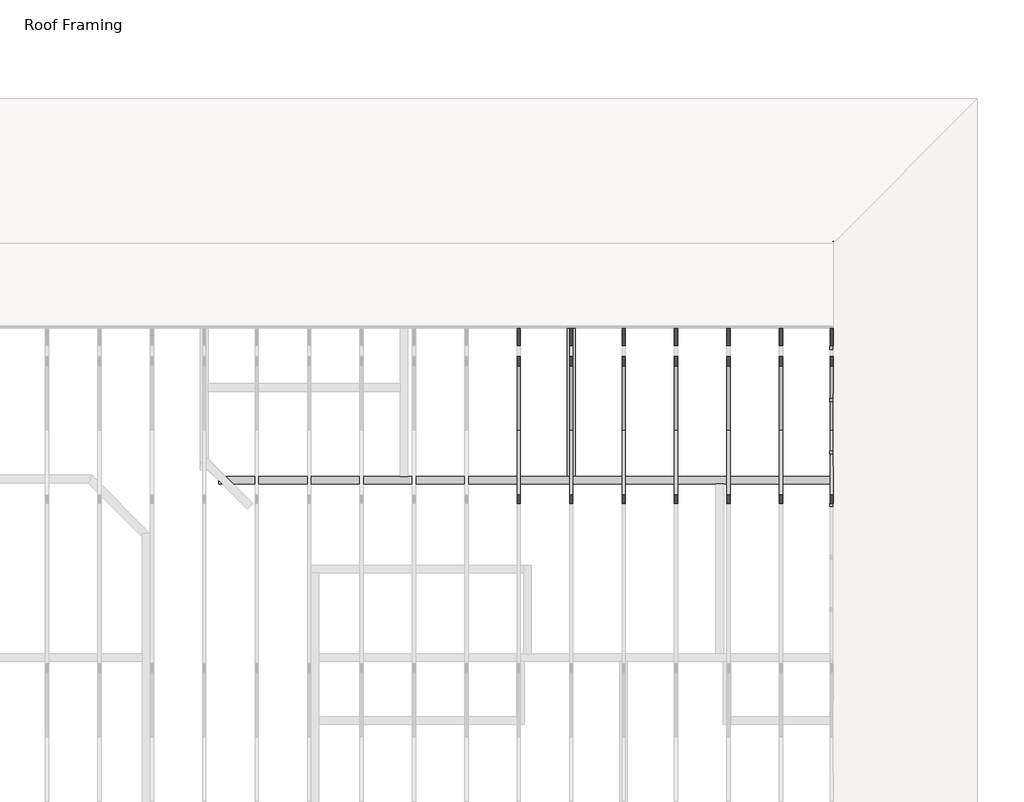
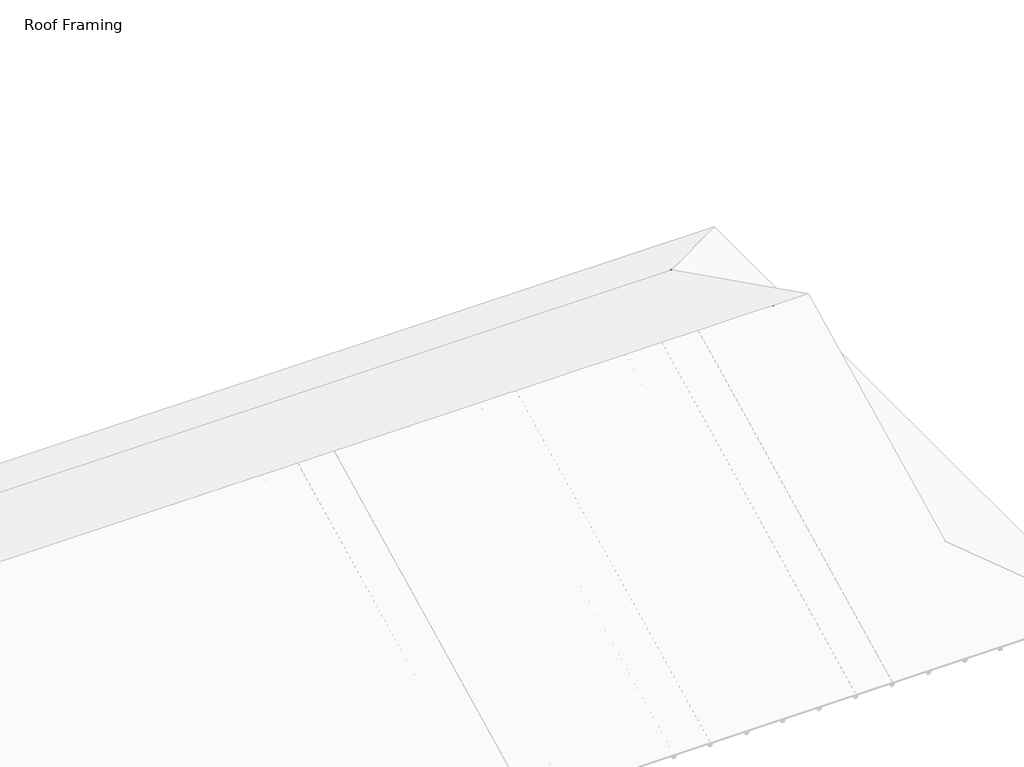
# One storey, part 7 of 7: 46 beams, 14 members.
"""IFC4 building model written with IfcOpenShell, lengths in millimetres."""

import ifcopenshell
import ifcopenshell.guid

model = None  # the IFC model being written
_history = None  # IfcOwnerHistory: only IFC2X3 demands one
_inside = {}  # id of a spatial element -> (the spatial element, [elements in it])
_under = {}  # id of a project, library or spatial element -> (it, [spatial elements below it])
_declared = {}  # id of a project -> (the project, [libraries it declares])
_typed = {}  # id of a type object -> (the type object, [elements of that type])
_made_of = {}  # id of a material, layer set ... -> (it, [elements and type objects made of it])


def new_model(schema):
    """Start an empty IFC model of exactly this schema.

    Asked for "IFC4X3", IfcOpenShell would pick the latest addendum, in which some entities
    have other attributes; the version numbers below select the first issue.
    IFC2X3 requires an IfcOwnerHistory on every rooted entity: one is made here for all.
    """
    global model, _history
    if schema == "IFC4X3":
        model = ifcopenshell.file(schema_version=(4, 3, 0, 0))
    else:
        model = ifcopenshell.file(schema=schema)
    _inside.clear()
    _under.clear()
    _declared.clear()
    _typed.clear()
    _made_of.clear()
    _history = None
    if model.schema == "IFC2X3":
        org = make("IfcOrganization", Name="unknown")
        user = make(
            "IfcPersonAndOrganization",
            ThePerson=make("IfcPerson", FamilyName="unknown"),
            TheOrganization=org,
        )
        app = make(
            "IfcApplication",
            ApplicationDeveloper=org,
            Version="unknown",
            ApplicationFullName="unknown",
            ApplicationIdentifier="unknown",
        )
        _history = make(
            "IfcOwnerHistory",
            OwningUser=user,
            OwningApplication=app,
            ChangeAction="ADDED",
            CreationDate=0,
        )
    return model


def make(cls, **values):
    """One entity of the class cls with the attributes given. An attribute that is None is left unset."""
    return model.create_entity(
        cls, **{name: value for name, value in values.items() if value is not None}
    )


def rooted(cls, **values):
    """An entity with a GlobalId (a new one), such as an element, a storey or a relation."""
    return make(cls, GlobalId=ifcopenshell.guid.new(), OwnerHistory=_history, **values)


def si_unit(unit_type, name, prefix=None):
    """IfcSIUnit, for example si_unit("LENGTHUNIT", "METRE", prefix="MILLI")."""
    return make("IfcSIUnit", UnitType=unit_type, Prefix=prefix, Name=name)


def assignment(units):
    """IfcUnitAssignment: the units of a project."""
    return None if units is None else make("IfcUnitAssignment", Units=units)


def point(xyz):
    """IfcCartesianPoint."""
    return None if xyz is None else make("IfcCartesianPoint", Coordinates=xyz)


def direction(xyz):
    """IfcDirection."""
    return None if xyz is None else make("IfcDirection", DirectionRatios=xyz)


def frame(location, z_axis=None, x_axis=None):
    """IfcAxis2Placement3D, a coordinate frame: its origin and axes. An axis left out is left unset."""
    return make(
        "IfcAxis2Placement3D",
        Location=point(location),
        Axis=direction(z_axis),
        RefDirection=direction(x_axis),
    )


def origin():
    """The frame at (0, 0, 0) with its axes left unset."""
    return frame((0.0, 0.0, 0.0))


def place(relative_to, where):
    """IfcLocalPlacement: puts the frame where relative to a parent placement (None: the world)."""
    return make(
        "IfcLocalPlacement", PlacementRelTo=relative_to, RelativePlacement=where
    )


def context(
    kind, dimensions, precision=None, world=None, true_north=None, identifier=None
):
    """IfcGeometricRepresentationContext, for example the 3D "Model" context."""
    return make(
        "IfcGeometricRepresentationContext",
        ContextIdentifier=identifier,
        ContextType=kind,
        CoordinateSpaceDimension=dimensions,
        Precision=precision,
        WorldCoordinateSystem=world,
        TrueNorth=true_north,
    )


def project(units=None, contexts=None):
    """IfcProject with its units and contexts."""
    return rooted(
        "IfcProject",
        Name="project",
        RepresentationContexts=contexts,
        UnitsInContext=assignment(units),
    )


def spatial(cls, under=None, at=None, **own):
    """A site, building, storey or space (cls), placed at a placement, below another one or the project."""
    s = rooted(cls, ObjectPlacement=at, **own)
    if under is not None:
        _under.setdefault(under.id(), (under, []))[1].append(s)
    return s


def polyline(points):
    """IfcPolyline through the points."""
    return make("IfcPolyline", Points=[point(p) for p in points])


def outline(outer, holes=None, kind="AREA"):
    """IfcArbitraryClosedProfileDef: a profile drawn as a closed curve; with holes, ...WithVoids."""
    if holes is None:
        return make("IfcArbitraryClosedProfileDef", ProfileType=kind, OuterCurve=outer)
    return make(
        "IfcArbitraryProfileDefWithVoids",
        ProfileType=kind,
        OuterCurve=outer,
        InnerCurves=holes,
    )


def extrude(swept, where, along, depth):
    """IfcExtrudedAreaSolid: the profile swept, set in the frame where, extruded along a direction by depth."""
    return make(
        "IfcExtrudedAreaSolid",
        SweptArea=swept,
        Position=where,
        ExtrudedDirection=direction(along),
        Depth=depth,
    )


def shape(context_of_items, identifier, shape_type, items):
    """IfcShapeRepresentation: the items that make up one representation, for example the "Body"."""
    return make(
        "IfcShapeRepresentation",
        ContextOfItems=context_of_items,
        RepresentationIdentifier=identifier,
        RepresentationType=shape_type,
        Items=items,
    )


def source(mapping_origin, context_of_items, identifier, shape_type, items):
    """IfcRepresentationMap: a shape defined once, which mapped items show again and again."""
    return make(
        "IfcRepresentationMap",
        MappingOrigin=mapping_origin,
        MappedRepresentation=shape(context_of_items, identifier, shape_type, items),
    )


def transform(
    local_origin,
    x_axis=None,
    y_axis=None,
    z_axis=None,
    scale=None,
    scale2=None,
    scale3=None,
    uniform=True,
):
    """IfcCartesianTransformationOperator3D, or its non-uniform kind. x_axis, y_axis, z_axis: its Axis1, 2, 3."""
    if uniform:
        return make(
            "IfcCartesianTransformationOperator3D",
            Axis1=direction(x_axis),
            Axis2=direction(y_axis),
            LocalOrigin=point(local_origin),
            Scale=scale,
            Axis3=direction(z_axis),
        )
    return make(
        "IfcCartesianTransformationOperator3DnonUniform",
        Axis1=direction(x_axis),
        Axis2=direction(y_axis),
        LocalOrigin=point(local_origin),
        Scale=scale,
        Axis3=direction(z_axis),
        Scale2=scale2,
        Scale3=scale3,
    )


def mapped(mapping_source, mapping_target):
    """IfcMappedItem: shows the shape of a source again, moved by a transform."""
    return make(
        "IfcMappedItem", MappingSource=mapping_source, MappingTarget=mapping_target
    )


def made_of(thing, what):
    """Note that an element or type object is made of a material, layer set ...; save() writes the relation."""
    if what is not None:
        _made_of.setdefault(what.id(), (what, []))[1].append(thing)
    return thing


def element(
    cls,
    number,
    at=None,
    inside=None,
    cuts=None,
    type_object=None,
    material=None,
    context=None,
    identifier="Body",
    shape_type=None,
    held_by="IfcProductDefinitionShape",
    body=None,
    shapes=None,
    **own,
):
    """One element of the class cls, such as IfcWall. Its Tag is "e" and its number.

    at: its placement. inside: the storey or other place that contains it. cuts: it is an
    opening in that element (IfcRelVoidsElement). A single representation is given by context,
    identifier, shape_type and body (its items); several are given by shapes. held_by: the class
    of the entity that holds the representations. save() writes the other relations.
    """
    e = rooted(cls, Tag="e%d" % number, ObjectPlacement=at, **own)
    if body is not None:
        shapes = [shape(context, identifier, shape_type, body)]
    if shapes is not None:
        e.Representation = make(held_by, Representations=shapes)
    if inside is not None:
        _inside.setdefault(inside.id(), (inside, []))[1].append(e)
    if cuts is not None:
        rooted(
            "IfcRelVoidsElement", RelatingBuildingElement=cuts, RelatedOpeningElement=e
        )
    if type_object is not None:
        _typed.setdefault(type_object.id(), (type_object, []))[1].append(e)
    return made_of(e, material)


def aggregate(whole, parts):
    """IfcRelAggregates: a whole, such as a stair, and the parts it consists of."""
    return rooted("IfcRelAggregates", RelatingObject=whole, RelatedObjects=parts)


def save(model, path):
    """Write the relations noted so far, then the file.

    IfcRelAggregates (storeys below a building ...), IfcRelContainedInSpatialStructure (elements
    in a storey), IfcRelDefinesByType, IfcRelAssociatesMaterial and IfcRelDeclares: one each for
    every whole, place, type object, material and project.
    """
    for whole, parts in _under.values():
        aggregate(whole, parts)
    for where, things in _inside.values():
        rooted(
            "IfcRelContainedInSpatialStructure",
            RelatedElements=things,
            RelatingStructure=where,
        )
    for kind, things in _typed.values():
        rooted("IfcRelDefinesByType", RelatedObjects=things, RelatingType=kind)
    for what, things in _made_of.values():
        rooted("IfcRelAssociatesMaterial", RelatedObjects=things, RelatingMaterial=what)
    for by, libraries in _declared.values():
        rooted("IfcRelDeclares", RelatingContext=by, RelatedDefinitions=libraries)
    model.write(path)


def dimension_lumber_72c26da1(model_context):
    return source(origin(), model_context, "Body", "SweptSolid", [
        extrude(outline(polyline([(927.1, 44.45), (927.1, -44.45), (-971.55, -44.45), (-971.55, 44.45), (927.1, 44.45)])), frame((0.0, 0.0, -19.05), z_axis=(0.0, 0.0, 1.0), x_axis=(1.0, 0.0, 0.0)), (0.0, 0.0, 1.0), 38.1),
    ])


def dimension_lumber_1b552245(model_context):
    return source(origin(), model_context, "Body", "SweptSolid", [
        extrude(outline(polyline([(1918.49375, 44.45), (1918.49375, -44.45), (-1918.49375, -44.45), (-1918.49375, 44.45), (1918.49375, 44.45)])), frame((0.0, 0.0, -19.05), z_axis=(0.0, 0.0, 1.0), x_axis=(1.0, 0.0, 0.0)), (0.0, 0.0, 1.0), 38.1),
    ])


def dimension_lumber_5c8890d8(model_context):
    return source(origin(), model_context, "Body", "SweptSolid", [
        extrude(outline(polyline([(330.0062925, 44.45), (330.0062925, -44.45), (-285.5562925, -44.45), (-285.5562925, 44.45), (330.0062925, 44.45)])), frame((0.0, 0.0, -19.05), z_axis=(0.0, 0.0, 1.0), x_axis=(1.0, 0.0, 0.0)), (0.0, 0.0, 1.0), 38.1),
    ])


def dimension_lumber_f00769ea(model_context):
    return source(origin(), model_context, "Body", "SweptSolid", [
        extrude(outline(polyline([(927.1, 44.45), (927.1, -44.45), (-1016.0, -44.45), (-1016.0, 44.45), (927.1, 44.45)])), frame((0.0, 0.0, -19.05), z_axis=(0.0, 0.0, 1.0), x_axis=(1.0, 0.0, 0.0)), (0.0, 0.0, 1.0), 38.1),
    ])


def dimension_lumber_39962a34(model_context):
    return source(origin(), model_context, "Body", "SweptSolid", [
        extrude(outline(polyline([(1941.5125, 44.45), (1941.5125, -44.45), (-1895.475, -44.45), (-1895.475, 44.45), (1941.5125, 44.45)])), frame((0.0, 0.0, -19.05), z_axis=(0.0, 0.0, 1.0), x_axis=(1.0, 0.0, 0.0)), (0.0, 0.0, 1.0), 38.1),
    ])


def dimension_lumber_4fd1e5d7(model_context):
    return source(origin(), model_context, "Body", "SweptSolid", [
        extrude(outline(polyline([(285.5562925, 44.45), (285.5562925, -44.45), (-330.0062925, -44.45), (-330.0062925, 44.45), (285.5562925, 44.45)])), frame((0.0, 0.0, -19.05), z_axis=(0.0, 0.0, 1.0), x_axis=(1.0, 0.0, 0.0)), (0.0, 0.0, 1.0), 38.1),
    ])


model = new_model("IFC4")

# Units and contexts
model_context = context("Model", 3, world=origin())
ifc_project = project(units=[si_unit("LENGTHUNIT", "METRE", prefix="MILLI")], contexts=[model_context])

# Site, building, storey
site = spatial("IfcSite", under=ifc_project)
building = spatial("IfcBuilding", under=site)
storey = spatial("IfcBuildingStorey", under=building, Name="Roof Framing", Elevation=2768.6)

# Beams
placement = place(None, origin())
element("IfcBeam", 1, ObjectType="Dimension Lumber : Roof Lumbers", at=placement, inside=storey, context=model_context, shape_type="SweptSolid", body=[
    extrude(outline(polyline([(0.0, -38.1), (0.0, 0.0), (1874.2721787, 0.0), (1874.2721787, -38.1), (0.0, -38.1)])), frame((13672.6274862, 213.0959053, 2554.840297), z_axis=(0.44721359549993345, 0.0, 0.8944271909999282), x_axis=(-0.8944271909999282, 0.0, 0.44721359549993345)), (0.0, 0.0, 1.0), 88.9),
    extrude(outline(polyline([(2554.840297, 13672.6274862), (2558.1548743, 13674.2847749), (2653.4048743, 13674.2847749), (3472.5548743, 12035.9847749), (3393.040297, 11996.2274862), (2554.840297, 13672.6274862)])), frame((0.0, 213.0959053, 0.0), z_axis=(0.0, 1.0, 0.0), x_axis=(0.0, 0.0, 1.0)), (0.0, 0.0, 1.0), 38.1),
    extrude(outline(polyline([(2554.840297, 13672.6274862), (2558.1548743, 13674.2847749), (2653.4048743, 13674.2847749), (3472.5548743, 12035.9847749), (3373.1616527, 12035.9847749), (2554.840297, 13672.6274862)])), frame((0.0, 213.0959053, 0.0), z_axis=(0.0, 1.0, 0.0), x_axis=(0.0, 0.0, 1.0)), (0.0, 0.0, 1.0), 38.1),
])
element("IfcBeam", 2, ObjectType="Dimension Lumber : Roof Lumbers", at=placement, inside=storey, context=model_context, shape_type="SweptSolid", body=[
    extrude(outline(polyline([(0.0, -38.1), (0.0, 0.0), (1874.2721787, 0.0), (1874.2721787, -38.1), (0.0, -38.1)])), frame((13672.6274862, 822.6959053, 2554.840297), z_axis=(0.44721359549993367, 0.0, 0.8944271909999281), x_axis=(-0.8944271909999281, 0.0, 0.44721359549993367)), (0.0, 0.0, 1.0), 88.9),
    extrude(outline(polyline([(2554.840297, 13672.6274862), (2558.1548743, 13674.2847749), (2653.4048743, 13674.2847749), (3472.5548743, 12035.9847749), (3393.040297, 11996.2274862), (2554.840297, 13672.6274862)])), frame((0.0, 822.6959053, 0.0), z_axis=(0.0, 1.0, 0.0), x_axis=(0.0, 0.0, 1.0)), (0.0, 0.0, 1.0), 38.1),
    extrude(outline(polyline([(2554.840297, 13672.6274862), (2558.1548743, 13674.2847749), (2653.4048743, 13674.2847749), (3472.5548743, 12035.9847749), (3373.1616527, 12035.9847749), (2554.840297, 13672.6274862)])), frame((0.0, 822.6959053, 0.0), z_axis=(0.0, 1.0, 0.0), x_axis=(0.0, 0.0, 1.0)), (0.0, 0.0, 1.0), 38.1),
])
element("IfcBeam", 3, ObjectType="Dimension Lumber : Roof Lumbers", at=placement, inside=storey, context=model_context, shape_type="SweptSolid", body=[
    extrude(outline(polyline([(0.0, -38.1), (0.0, 0.0), (1874.2721787, 0.0), (1874.2721787, -38.1), (0.0, -38.1)])), frame((13672.6274862, 1432.2959053, 2554.840297), z_axis=(0.44721359549993367, 0.0, 0.8944271909999281), x_axis=(-0.8944271909999281, 0.0, 0.44721359549993367)), (0.0, 0.0, 1.0), 88.9),
    extrude(outline(polyline([(2554.840297, 13672.6274862), (2558.1548743, 13674.2847749), (2653.4048743, 13674.2847749), (3472.5548743, 12035.9847749), (3393.040297, 11996.2274862), (2554.840297, 13672.6274862)])), frame((0.0, 1432.2959053, 0.0), z_axis=(0.0, 1.0, 0.0), x_axis=(0.0, 0.0, 1.0)), (0.0, 0.0, 1.0), 38.1),
    extrude(outline(polyline([(2554.840297, 13672.6274862), (2558.1548743, 13674.2847749), (2653.4048743, 13674.2847749), (3472.5548743, 12035.9847749), (3373.1616527, 12035.9847749), (2554.840297, 13672.6274862)])), frame((0.0, 1432.2959053, 0.0), z_axis=(0.0, 1.0, 0.0), x_axis=(0.0, 0.0, 1.0)), (0.0, 0.0, 1.0), 38.1),
])
element("IfcBeam", 4, ObjectType="Dimension Lumber : Roof Lumbers", at=placement, inside=storey, context=model_context, shape_type="SweptSolid", body=[
    extrude(outline(polyline([(0.0, -38.1), (0.0, 0.0), (1874.2721787, 0.0), (1874.2721787, -38.1), (0.0, -38.1)])), frame((13672.6274862, 2041.8959053, 2554.840297), z_axis=(0.44721359549993345, 0.0, 0.8944271909999282), x_axis=(-0.8944271909999282, 0.0, 0.44721359549993345)), (0.0, 0.0, 1.0), 88.9),
    extrude(outline(polyline([(2554.840297, 13672.6274862), (2558.1548743, 13674.2847749), (2653.4048743, 13674.2847749), (3472.5548743, 12035.9847749), (3393.040297, 11996.2274862), (2554.840297, 13672.6274862)])), frame((0.0, 2041.8959053, 0.0), z_axis=(0.0, 1.0, 0.0), x_axis=(0.0, 0.0, 1.0)), (0.0, 0.0, 1.0), 38.1),
    extrude(outline(polyline([(2554.840297, 13672.6274862), (2558.1548743, 13674.2847749), (2653.4048743, 13674.2847749), (3472.5548743, 12035.9847749), (3373.1616527, 12035.9847749), (2554.840297, 13672.6274862)])), frame((0.0, 2041.8959053, 0.0), z_axis=(0.0, 1.0, 0.0), x_axis=(0.0, 0.0, 1.0)), (0.0, 0.0, 1.0), 38.1),
])
element("IfcBeam", 5, ObjectType="Dimension Lumber : Roof Lumbers", at=placement, inside=storey, context=model_context, shape_type="SweptSolid", body=[
    extrude(outline(polyline([(0.0, -38.1), (0.0, 0.0), (1874.2721787, 0.0), (1874.2721787, -38.1), (0.0, -38.1)])), frame((13672.6274862, 2651.4959053, 2554.840297), z_axis=(0.44721359549993367, 0.0, 0.8944271909999281), x_axis=(-0.8944271909999281, 0.0, 0.44721359549993367)), (0.0, 0.0, 1.0), 88.9),
    extrude(outline(polyline([(2554.840297, 13672.6274862), (2558.1548743, 13674.2847749), (2653.4048743, 13674.2847749), (3472.5548743, 12035.9847749), (3393.040297, 11996.2274862), (2554.840297, 13672.6274862)])), frame((0.0, 2651.4959053, 0.0), z_axis=(0.0, 1.0, 0.0), x_axis=(0.0, 0.0, 1.0)), (0.0, 0.0, 1.0), 38.1),
    extrude(outline(polyline([(2554.840297, 13672.6274862), (2558.1548743, 13674.2847749), (2653.4048743, 13674.2847749), (3472.5548743, 12035.9847749), (3373.1616527, 12035.9847749), (2554.840297, 13672.6274862)])), frame((0.0, 2651.4959053, 0.0), z_axis=(0.0, 1.0, 0.0), x_axis=(0.0, 0.0, 1.0)), (0.0, 0.0, 1.0), 38.1),
])
element("IfcBeam", 6, ObjectType="Dimension Lumber : Roof Lumbers", at=placement, inside=storey, context=model_context, shape_type="SweptSolid", body=[
    extrude(outline(polyline([(0.0, -38.1), (0.0, 0.0), (1877.070187, 0.0), (1877.070187, -38.1), (0.0, -38.1)])), frame((13672.6274862, 3261.0959053, 2554.840297), z_axis=(0.44721359549993367, 0.0, 0.8944271909999281), x_axis=(-0.8944271909999281, 0.0, 0.44721359549993367)), (0.0, 0.0, 1.0), 88.9),
    extrude(outline(polyline([(2554.840297, 13672.6274862), (2558.1548743, 13674.2847749), (2653.4048743, 13674.2847749), (3473.8061816, 12033.4821602), (3394.2916044, 11993.7248716), (2554.840297, 13672.6274862)])), frame((0.0, 3261.0959053, 0.0), z_axis=(0.0, 1.0, 0.0), x_axis=(0.0, 0.0, 1.0)), (0.0, 0.0, 1.0), 38.1),
    extrude(outline(polyline([(2554.840297, 13672.6274862), (2558.1548743, 13674.2847749), (2653.4048743, 13674.2847749), (3472.5548743, 12035.9847749), (3373.1616527, 12035.9847749), (2554.840297, 13672.6274862)])), frame((0.0, 3261.0959053, 0.0), z_axis=(0.0, 1.0, 0.0), x_axis=(0.0, 0.0, 1.0)), (0.0, 0.0, 1.0), 38.1),
])
element("IfcBeam", 7, ObjectType="Dimension Lumber : Roof Lumbers", at=placement, inside=storey, context=model_context, shape_type="SweptSolid", body=[
    extrude(outline(polyline([(12035.9847749, 251.1959053), (13244.0722749, 251.1959053), (13244.0722749, 213.0959053), (12035.9847749, 213.0959053), (12035.9847749, 251.1959053)])), frame((0.0, 0.0, 2768.6), z_axis=(0.0, 0.0, 1.0), x_axis=(1.0, 0.0, 0.0)), (0.0, 0.0, 1.0), 88.9),
    extrude(outline(polyline([(2768.6, 12035.9847749), (2768.6, 13244.0722749), (2769.1179027, 13244.0722749), (2857.5, 13067.3080803), (2857.5, 12035.9847749), (2768.6, 12035.9847749)])), frame((0.0, 213.0959053, 0.0), z_axis=(0.0, 1.0, 0.0), x_axis=(0.0, 0.0, 1.0)), (0.0, 0.0, 1.0), 38.1),
])
element("IfcBeam", 8, ObjectType="Dimension Lumber : Roof Lumbers", at=placement, inside=storey, context=model_context, shape_type="SweptSolid", body=[
    extrude(outline(polyline([(12035.9847749, 860.7959053), (13244.0722749, 860.7959053), (13244.0722749, 822.6959053), (12035.9847749, 822.6959053), (12035.9847749, 860.7959053)])), frame((0.0, 0.0, 2768.6), z_axis=(0.0, 0.0, 1.0), x_axis=(1.0, 0.0, 0.0)), (0.0, 0.0, 1.0), 88.9),
    extrude(outline(polyline([(2768.6, 12035.9847749), (2768.6, 13244.0722749), (2769.1179027, 13244.0722749), (2857.5, 13067.3080803), (2857.5, 12035.9847749), (2768.6, 12035.9847749)])), frame((0.0, 822.6959053, 0.0), z_axis=(0.0, 1.0, 0.0), x_axis=(0.0, 0.0, 1.0)), (0.0, 0.0, 1.0), 38.1),
])
element("IfcBeam", 9, ObjectType="Dimension Lumber : Roof Lumbers", at=placement, inside=storey, context=model_context, shape_type="SweptSolid", body=[
    extrude(outline(polyline([(12035.9847749, 1470.3959053), (13244.0722749, 1470.3959053), (13244.0722749, 1432.2959053), (12035.9847749, 1432.2959053), (12035.9847749, 1470.3959053)])), frame((0.0, 0.0, 2768.6), z_axis=(0.0, 0.0, 1.0), x_axis=(1.0, 0.0, 0.0)), (0.0, 0.0, 1.0), 88.9),
    extrude(outline(polyline([(2768.6, 12035.9847749), (2768.6, 13244.0722749), (2769.1179027, 13244.0722749), (2857.5, 13067.3080803), (2857.5, 12035.9847749), (2768.6, 12035.9847749)])), frame((0.0, 1432.2959053, 0.0), z_axis=(0.0, 1.0, 0.0), x_axis=(0.0, 0.0, 1.0)), (0.0, 0.0, 1.0), 38.1),
])
element("IfcBeam", 10, ObjectType="Dimension Lumber : Roof Lumbers", at=placement, inside=storey, context=model_context, shape_type="SweptSolid", body=[
    extrude(outline(polyline([(12035.9847749, 2079.9959053), (13244.0722749, 2079.9959053), (13244.0722749, 2041.8959053), (12035.9847749, 2041.8959053), (12035.9847749, 2079.9959053)])), frame((0.0, 0.0, 2768.6), z_axis=(0.0, 0.0, 1.0), x_axis=(1.0, 0.0, 0.0)), (0.0, 0.0, 1.0), 88.9),
    extrude(outline(polyline([(2768.6, 12035.9847749), (2768.6, 13244.0722749), (2769.1179027, 13244.0722749), (2857.5, 13067.3080803), (2857.5, 12035.9847749), (2768.6, 12035.9847749)])), frame((0.0, 2041.8959053, 0.0), z_axis=(0.0, 1.0, 0.0), x_axis=(0.0, 0.0, 1.0)), (0.0, 0.0, 1.0), 38.1),
])
element("IfcBeam", 11, ObjectType="Dimension Lumber : Roof Lumbers", at=placement, inside=storey, context=model_context, shape_type="SweptSolid", body=[
    extrude(outline(polyline([(12035.9847749, 2689.5959053), (13244.0722749, 2689.5959053), (13244.0722749, 2651.4959053), (12035.9847749, 2651.4959053), (12035.9847749, 2689.5959053)])), frame((0.0, 0.0, 2768.6), z_axis=(0.0, 0.0, 1.0), x_axis=(1.0, 0.0, 0.0)), (0.0, 0.0, 1.0), 88.9),
    extrude(outline(polyline([(2768.6, 12035.9847749), (2768.6, 13244.0722749), (2769.1179027, 13244.0722749), (2857.5, 13067.3080803), (2857.5, 12035.9847749), (2768.6, 12035.9847749)])), frame((0.0, 2651.4959053, 0.0), z_axis=(0.0, 1.0, 0.0), x_axis=(0.0, 0.0, 1.0)), (0.0, 0.0, 1.0), 38.1),
])
element("IfcBeam", 12, ObjectType="Dimension Lumber : Roof Lumbers", at=placement, inside=storey, context=model_context, shape_type="SweptSolid", body=[
    extrude(outline(polyline([(12035.9847749, 3299.1959053), (13244.0722749, 3299.1959053), (13244.0722749, 3261.0959053), (12035.9847749, 3261.0959053), (12035.9847749, 3299.1959053)])), frame((0.0, 0.0, 2768.6), z_axis=(0.0, 0.0, 1.0), x_axis=(1.0, 0.0, 0.0)), (0.0, 0.0, 1.0), 88.9),
    extrude(outline(polyline([(2768.6, 12035.9847749), (2768.6, 13244.0722749), (2769.1179027, 13244.0722749), (2857.5, 13067.3080803), (2857.5, 12035.9847749), (2768.6, 12035.9847749)])), frame((0.0, 3261.0959053, 0.0), z_axis=(0.0, 1.0, 0.0), x_axis=(0.0, 0.0, 1.0)), (0.0, 0.0, 1.0), 38.1),
])
element("IfcBeam", 13, ObjectType="Dimension Lumber : Top Supporting Lumbers", at=placement, inside=storey, context=model_context, shape_type="SweptSolid", body=[
    extrude(outline(polyline([(13155.1722749, 562.3459053), (13155.1722749, 473.4459053), (4885.8847749, 473.4459053), (4885.8847749, 562.3459053), (13155.1722749, 562.3459053)])), frame((0.0, 0.0, 2692.4), z_axis=(0.0, 0.0, 1.0), x_axis=(1.0, 0.0, 0.0)), (0.0, 0.0, 1.0), 38.1),
    extrude(outline(polyline([(13155.1722749, 562.3459053), (13155.1722749, 473.4459053), (4930.3347749, 473.4459053), (4967.1583606, 562.3459053), (13155.1722749, 562.3459053)])), frame((0.0, 0.0, 2692.4), z_axis=(0.0, 0.0, 1.0), x_axis=(1.0, 0.0, 0.0)), (0.0, 0.0, 1.0), 38.1),
])
element("IfcBeam", 14, ObjectType="Dimension Lumber : Top Supporting Lumbers", at=placement, inside=storey, context=model_context, shape_type="SweptSolid", body=[
    extrude(outline(polyline([(4885.8847749, 473.4459053), (4885.8847749, 562.3459053), (13155.1722749, 562.3459053), (13155.1722749, 473.4459053), (4885.8847749, 473.4459053)])), frame((0.0, 0.0, 2730.5), z_axis=(0.0, 0.0, 1.0), x_axis=(1.0, 0.0, 0.0)), (0.0, 0.0, 1.0), 38.1),
    extrude(outline(polyline([(4967.1583606, 562.3459053), (13155.1722749, 562.3459053), (13155.1722749, 473.4459053), (4930.3347749, 473.4459053), (4967.1583606, 562.3459053)])), frame((0.0, 0.0, 2730.5), z_axis=(0.0, 0.0, 1.0), x_axis=(1.0, 0.0, 0.0)), (0.0, 0.0, 1.0), 38.1),
])
dimension_lumber_shape = dimension_lumber_72c26da1(model_context)
element("IfcBeam", 15, ObjectType="Dimension Lumber : Top Supporting Lumbers", at=placement, inside=storey, context=model_context, shape_type="MappedRepresentation", body=[
    mapped(dimension_lumber_shape, transform((8016.4347749, 2753.0959053, 2711.45), x_axis=(1.0, 0.0, 0.0), y_axis=(0.0, 1.0, 0.0), z_axis=(0.0, 0.0, 1.0))),
])
dimension_lumber_2_shape = dimension_lumber_1b552245(model_context)
element("IfcBeam", 16, ObjectType="Dimension Lumber : Top Supporting Lumbers", at=placement, inside=storey, context=model_context, shape_type="MappedRepresentation", body=[
    mapped(dimension_lumber_2_shape, transform((8987.9847749, 2480.8396553, 2711.45), x_axis=(0.0, 1.0, 0.0), y_axis=(-1.0, 0.0, 0.0), z_axis=(0.0, 0.0, 1.0))),
])
dimension_lumber_3_shape = dimension_lumber_5c8890d8(model_context)
element("IfcBeam", 17, ObjectType="Dimension Lumber : Top Supporting Lumbers", at=placement, inside=storey, context=model_context, shape_type="MappedRepresentation", body=[
    mapped(dimension_lumber_3_shape, transform((7698.9347749, 4113.7771128, 2711.45), x_axis=(0.0, -1.0, 0.0), y_axis=(1.0, 0.0, 0.0), z_axis=(0.0, 0.0, 1.0))),
])
dimension_lumber_4_shape = dimension_lumber_f00769ea(model_context)
element("IfcBeam", 18, ObjectType="Dimension Lumber : Top Supporting Lumbers", at=placement, inside=storey, context=model_context, shape_type="MappedRepresentation", body=[
    mapped(dimension_lumber_4_shape, transform((8016.4347749, 2753.0959053, 2749.55), x_axis=(1.0, 0.0, 0.0), y_axis=(0.0, 1.0, 0.0), z_axis=(0.0, 0.0, 1.0))),
])
dimension_lumber_5_shape = dimension_lumber_39962a34(model_context)
element("IfcBeam", 19, ObjectType="Dimension Lumber : Top Supporting Lumbers", at=placement, inside=storey, context=model_context, shape_type="MappedRepresentation", body=[
    mapped(dimension_lumber_5_shape, transform((8987.9847749, 2457.8209053, 2749.55), x_axis=(0.0, 1.0, 0.0), y_axis=(-1.0, 0.0, 0.0), z_axis=(0.0, 0.0, 1.0))),
])
dimension_lumber_6_shape = dimension_lumber_4fd1e5d7(model_context)
element("IfcBeam", 20, ObjectType="Dimension Lumber : Top Supporting Lumbers", at=placement, inside=storey, context=model_context, shape_type="MappedRepresentation", body=[
    mapped(dimension_lumber_6_shape, transform((7698.9347749, 4113.7771128, 2749.55), x_axis=(0.0, 1.0, 0.0), y_axis=(-1.0, 0.0, 0.0), z_axis=(0.0, 0.0, 1.0))),
])
element("IfcBeam", 21, ObjectType="Dimension Lumber : 2x4 Blocking", at=placement, inside=storey, context=model_context, shape_type="SweptSolid", body=[
    extrude(outline(polyline([(13674.2847749, 213.0959053), (13293.2847749, 213.0959053), (13293.2847749, 251.1959053), (13674.2847749, 251.1959053), (13674.2847749, 213.0959053)])), frame((0.0, 0.0, 2564.60625), z_axis=(0.0, 0.0, 1.0), x_axis=(1.0, 0.0, 0.0)), (0.0, 0.0, 1.0), 88.9),
    extrude(outline(polyline([(2653.50625, 13475.2955803), (2653.50625, 13293.2847749), (2564.60625, 13293.2847749), (2564.60625, 13653.0955803), (2653.50625, 13475.2955803)])), frame((0.0, 213.0959053, 0.0), z_axis=(0.0, 1.0, 0.0), x_axis=(0.0, 0.0, 1.0)), (0.0, 0.0, 1.0), 38.1),
])
element("IfcBeam", 22, ObjectType="Dimension Lumber : 2x4 Blocking", at=placement, inside=storey, context=model_context, shape_type="SweptSolid", body=[
    extrude(outline(polyline([(13674.2847749, 822.6959053), (13293.2847749, 822.6959053), (13293.2847749, 860.7959053), (13674.2847749, 860.7959053), (13674.2847749, 822.6959053)])), frame((0.0, 0.0, 2564.60625), z_axis=(0.0, 0.0, 1.0), x_axis=(1.0, 0.0, 0.0)), (0.0, 0.0, 1.0), 88.9),
    extrude(outline(polyline([(2653.50625, 13475.2955803), (2653.50625, 13293.2847749), (2564.60625, 13293.2847749), (2564.60625, 13653.0955803), (2653.50625, 13475.2955803)])), frame((0.0, 822.6959053, 0.0), z_axis=(0.0, 1.0, 0.0), x_axis=(0.0, 0.0, 1.0)), (0.0, 0.0, 1.0), 38.1),
])
element("IfcBeam", 23, ObjectType="Dimension Lumber : 2x4 Blocking", at=placement, inside=storey, context=model_context, shape_type="SweptSolid", body=[
    extrude(outline(polyline([(13674.2847749, 1432.2959053), (13293.2847749, 1432.2959053), (13293.2847749, 1470.3959053), (13674.2847749, 1470.3959053), (13674.2847749, 1432.2959053)])), frame((0.0, 0.0, 2564.60625), z_axis=(0.0, 0.0, 1.0), x_axis=(1.0, 0.0, 0.0)), (0.0, 0.0, 1.0), 88.9),
    extrude(outline(polyline([(2653.50625, 13475.2955803), (2653.50625, 13293.2847749), (2564.60625, 13293.2847749), (2564.60625, 13653.0955803), (2653.50625, 13475.2955803)])), frame((0.0, 1432.2959053, 0.0), z_axis=(0.0, 1.0, 0.0), x_axis=(0.0, 0.0, 1.0)), (0.0, 0.0, 1.0), 38.1),
])
element("IfcBeam", 24, ObjectType="Dimension Lumber : 2x4 Blocking", at=placement, inside=storey, context=model_context, shape_type="SweptSolid", body=[
    extrude(outline(polyline([(13674.2847749, 2041.8959053), (13293.2847749, 2041.8959053), (13293.2847749, 2079.9959053), (13674.2847749, 2079.9959053), (13674.2847749, 2041.8959053)])), frame((0.0, 0.0, 2564.60625), z_axis=(0.0, 0.0, 1.0), x_axis=(1.0, 0.0, 0.0)), (0.0, 0.0, 1.0), 88.9),
    extrude(outline(polyline([(2653.50625, 13475.2955803), (2653.50625, 13293.2847749), (2564.60625, 13293.2847749), (2564.60625, 13653.0955803), (2653.50625, 13475.2955803)])), frame((0.0, 2041.8959053, 0.0), z_axis=(0.0, 1.0, 0.0), x_axis=(0.0, 0.0, 1.0)), (0.0, 0.0, 1.0), 38.1),
])
element("IfcBeam", 25, ObjectType="Dimension Lumber : 2x4 Blocking", at=placement, inside=storey, context=model_context, shape_type="SweptSolid", body=[
    extrude(outline(polyline([(13674.2847749, 2651.4959053), (13293.2847749, 2651.4959053), (13293.2847749, 2689.5959053), (13674.2847749, 2689.5959053), (13674.2847749, 2651.4959053)])), frame((0.0, 0.0, 2564.60625), z_axis=(0.0, 0.0, 1.0), x_axis=(1.0, 0.0, 0.0)), (0.0, 0.0, 1.0), 88.9),
    extrude(outline(polyline([(2653.50625, 13475.2955803), (2653.50625, 13293.2847749), (2564.60625, 13293.2847749), (2564.60625, 13653.0955803), (2653.50625, 13475.2955803)])), frame((0.0, 2651.4959053, 0.0), z_axis=(0.0, 1.0, 0.0), x_axis=(0.0, 0.0, 1.0)), (0.0, 0.0, 1.0), 38.1),
])
element("IfcBeam", 26, ObjectType="Dimension Lumber : 2x4 Blocking", at=placement, inside=storey, context=model_context, shape_type="SweptSolid", body=[
    extrude(outline(polyline([(13674.2847749, 3261.0959053), (13293.2847749, 3261.0959053), (13293.2847749, 3299.1959053), (13674.2847749, 3299.1959053), (13674.2847749, 3261.0959053)])), frame((0.0, 0.0, 2564.60625), z_axis=(0.0, 0.0, 1.0), x_axis=(1.0, 0.0, 0.0)), (0.0, 0.0, 1.0), 88.9),
    extrude(outline(polyline([(2653.50625, 13475.2955803), (2653.50625, 13293.2847749), (2564.60625, 13293.2847749), (2564.60625, 13653.0955803), (2653.50625, 13475.2955803)])), frame((0.0, 3261.0959053, 0.0), z_axis=(0.0, 1.0, 0.0), x_axis=(0.0, 0.0, 1.0)), (0.0, 0.0, 1.0), 38.1),
])
element("IfcBeam", 27, ObjectType="Dimension Lumber : 2x4 Blocking", at=placement, inside=storey, context=model_context, shape_type="SweptSolid", body=[
    extrude(outline(polyline([(12035.9847749, 4918.4459053), (12035.9847749, 4537.4459053), (11997.8847749, 4537.4459053), (11997.8847749, 4918.4459053), (12035.9847749, 4918.4459053)])), frame((0.0, 0.0, 2564.60625), z_axis=(0.0, 0.0, 1.0), x_axis=(1.0, 0.0, 0.0)), (0.0, 0.0, 1.0), 88.9),
    extrude(outline(polyline([(4897.2567107, 2564.60625), (4537.4459053, 2564.60625), (4537.4459053, 2653.50625), (4719.4567107, 2653.50625), (4897.2567107, 2564.60625)])), frame((11997.8847749, 0.0, 0.0), z_axis=(1.0, 0.0, 0.0), x_axis=(0.0, 1.0, 0.0)), (0.0, 0.0, 1.0), 38.1),
])
element("IfcBeam", 28, ObjectType="Dimension Lumber : 2x4 Blocking", at=placement, inside=storey, context=model_context, shape_type="SweptSolid", body=[
    extrude(outline(polyline([(11445.4347749, 4918.4459053), (11445.4347749, 4537.4459053), (11407.3347749, 4537.4459053), (11407.3347749, 4918.4459053), (11445.4347749, 4918.4459053)])), frame((0.0, 0.0, 2564.60625), z_axis=(0.0, 0.0, 1.0), x_axis=(1.0, 0.0, 0.0)), (0.0, 0.0, 1.0), 88.9),
    extrude(outline(polyline([(4897.2567107, 2564.60625), (4537.4459053, 2564.60625), (4537.4459053, 2653.50625), (4719.4567107, 2653.50625), (4897.2567107, 2564.60625)])), frame((11407.3347749, 0.0, 0.0), z_axis=(1.0, 0.0, 0.0), x_axis=(0.0, 1.0, 0.0)), (0.0, 0.0, 1.0), 38.1),
])
element("IfcBeam", 29, ObjectType="Dimension Lumber : 2x4 Blocking", at=placement, inside=storey, context=model_context, shape_type="SweptSolid", body=[
    extrude(outline(polyline([(10835.8347749, 4918.4459053), (10835.8347749, 4537.4459053), (10797.7347749, 4537.4459053), (10797.7347749, 4918.4459053), (10835.8347749, 4918.4459053)])), frame((0.0, 0.0, 2564.60625), z_axis=(0.0, 0.0, 1.0), x_axis=(1.0, 0.0, 0.0)), (0.0, 0.0, 1.0), 88.9),
    extrude(outline(polyline([(4897.2567107, 2564.60625), (4537.4459053, 2564.60625), (4537.4459053, 2653.50625), (4719.4567107, 2653.50625), (4897.2567107, 2564.60625)])), frame((10797.7347749, 0.0, 0.0), z_axis=(1.0, 0.0, 0.0), x_axis=(0.0, 1.0, 0.0)), (0.0, 0.0, 1.0), 38.1),
])
element("IfcBeam", 30, ObjectType="Dimension Lumber : 2x4 Blocking", at=placement, inside=storey, context=model_context, shape_type="SweptSolid", body=[
    extrude(outline(polyline([(10226.2347749, 4918.4459053), (10226.2347749, 4537.4459053), (10188.1347749, 4537.4459053), (10188.1347749, 4918.4459053), (10226.2347749, 4918.4459053)])), frame((0.0, 0.0, 2564.60625), z_axis=(0.0, 0.0, 1.0), x_axis=(1.0, 0.0, 0.0)), (0.0, 0.0, 1.0), 88.9),
    extrude(outline(polyline([(4897.2567107, 2564.60625), (4537.4459053, 2564.60625), (4537.4459053, 2653.50625), (4719.4567107, 2653.50625), (4897.2567107, 2564.60625)])), frame((10188.1347749, 0.0, 0.0), z_axis=(1.0, 0.0, 0.0), x_axis=(0.0, 1.0, 0.0)), (0.0, 0.0, 1.0), 38.1),
])
element("IfcBeam", 31, ObjectType="Dimension Lumber : 2x4 Blocking", at=placement, inside=storey, context=model_context, shape_type="SweptSolid", body=[
    extrude(outline(polyline([(9616.6347749, 4918.4459053), (9616.6347749, 4537.4459053), (9578.5347749, 4537.4459053), (9578.5347749, 4918.4459053), (9616.6347749, 4918.4459053)])), frame((0.0, 0.0, 2564.60625), z_axis=(0.0, 0.0, 1.0), x_axis=(1.0, 0.0, 0.0)), (0.0, 0.0, 1.0), 88.9),
    extrude(outline(polyline([(4897.2567107, 2564.60625), (4537.4459053, 2564.60625), (4537.4459053, 2653.50625), (4719.4567107, 2653.50625), (4897.2567107, 2564.60625)])), frame((9578.5347749, 0.0, 0.0), z_axis=(1.0, 0.0, 0.0), x_axis=(0.0, 1.0, 0.0)), (0.0, 0.0, 1.0), 38.1),
])
element("IfcBeam", 32, ObjectType="Dimension Lumber : 2x4 Blocking", at=placement, inside=storey, context=model_context, shape_type="SweptSolid", body=[
    extrude(outline(polyline([(9007.0347749, 4918.4459053), (9007.0347749, 4537.4459053), (8968.9347749, 4537.4459053), (8968.9347749, 4918.4459053), (9007.0347749, 4918.4459053)])), frame((0.0, 0.0, 2564.60625), z_axis=(0.0, 0.0, 1.0), x_axis=(1.0, 0.0, 0.0)), (0.0, 0.0, 1.0), 88.9),
    extrude(outline(polyline([(4897.2567107, 2564.60625), (4537.4459053, 2564.60625), (4537.4459053, 2653.50625), (4719.4567107, 2653.50625), (4897.2567107, 2564.60625)])), frame((8968.9347749, 0.0, 0.0), z_axis=(1.0, 0.0, 0.0), x_axis=(0.0, 1.0, 0.0)), (0.0, 0.0, 1.0), 38.1),
])
element("IfcBeam", 33, ObjectType="Dimension Lumber : 2x4 Blocking", at=placement, inside=storey, context=model_context, shape_type="SweptSolid", body=[
    extrude(outline(polyline([(8397.4347749, 4918.4459053), (8397.4347749, 4537.4459053), (8359.3347749, 4537.4459053), (8359.3347749, 4918.4459053), (8397.4347749, 4918.4459053)])), frame((0.0, 0.0, 2564.60625), z_axis=(0.0, 0.0, 1.0), x_axis=(1.0, 0.0, 0.0)), (0.0, 0.0, 1.0), 88.9),
    extrude(outline(polyline([(4897.2567107, 2564.60625), (4537.4459053, 2564.60625), (4537.4459053, 2653.50625), (4719.4567107, 2653.50625), (4897.2567107, 2564.60625)])), frame((8359.3347749, 0.0, 0.0), z_axis=(1.0, 0.0, 0.0), x_axis=(0.0, 1.0, 0.0)), (0.0, 0.0, 1.0), 38.1),
])
element("IfcBeam", 34, ObjectType="Dimension Lumber : 2x4 Blocking", at=placement, inside=storey, context=model_context, shape_type="SweptSolid", body=[
    extrude(outline(polyline([(12423.3347749, 4537.4459053), (12423.3347749, 4907.7499323), (12461.4347749, 4907.7499323), (12461.4347749, 4537.4459053), (12423.3347749, 4537.4459053)])), frame((0.0, 0.0, 2564.60625), z_axis=(0.0, 0.0, 1.0), x_axis=(1.0, 0.0, 0.0)), (0.0, 0.0, 1.0), 88.9),
    extrude(outline(polyline([(4537.4459053, 2653.50625), (4719.4567107, 2653.50625), (4897.2567107, 2564.60625), (4537.4459053, 2564.60625), (4537.4459053, 2653.50625)])), frame((12423.3347749, 0.0, 0.0), z_axis=(1.0, 0.0, 0.0), x_axis=(0.0, 1.0, 0.0)), (0.0, 0.0, 1.0), 38.1),
])
element("IfcBeam", 35, ObjectType="Dimension Lumber : 2x4 Blocking", at=placement, inside=storey, context=model_context, shape_type="SweptSolid", body=[
    extrude(outline(polyline([(12829.7347749, 4537.4459053), (12829.7347749, 4918.4459053), (12867.8347749, 4918.4459053), (12867.8347749, 4537.4459053), (12829.7347749, 4537.4459053)])), frame((0.0, 0.0, 2564.60625), z_axis=(0.0, 0.0, 1.0), x_axis=(1.0, 0.0, 0.0)), (0.0, 0.0, 1.0), 88.9),
    extrude(outline(polyline([(4537.4459053, 2653.50625), (4719.4567107, 2653.50625), (4897.2567107, 2564.60625), (4537.4459053, 2564.60625), (4537.4459053, 2653.50625)])), frame((12829.7347749, 0.0, 0.0), z_axis=(1.0, 0.0, 0.0), x_axis=(0.0, 1.0, 0.0)), (0.0, 0.0, 1.0), 38.1),
])
element("IfcBeam", 36, ObjectType="Dimension Lumber : 2x4 Blocking", at=placement, inside=storey, context=model_context, shape_type="SweptSolid", body=[
    extrude(outline(polyline([(13274.2347749, 4918.4459053), (13274.2347749, 4537.4459053), (13236.1347749, 4537.4459053), (13236.1347749, 4918.4459053), (13274.2347749, 4918.4459053)])), frame((0.0, 0.0, 2564.60625), z_axis=(0.0, 0.0, 1.0), x_axis=(1.0, 0.0, 0.0)), (0.0, 0.0, 1.0), 88.9),
    extrude(outline(polyline([(4897.2567107, 2564.60625), (4537.4459053, 2564.60625), (4537.4459053, 2653.50625), (4719.4567107, 2653.50625), (4897.2567107, 2564.60625)])), frame((13236.1347749, 0.0, 0.0), z_axis=(1.0, 0.0, 0.0), x_axis=(0.0, 1.0, 0.0)), (0.0, 0.0, 1.0), 38.1),
])
element("IfcBeam", 37, ObjectType="Dimension Lumber : 2x4 Blocking", at=placement, inside=storey, context=model_context, shape_type="SweptSolid", body=[
    extrude(outline(polyline([(13674.2847749, 3667.4959053), (13293.2847749, 3667.4959053), (13293.2847749, 3705.5959053), (13674.2847749, 3705.5959053), (13674.2847749, 3667.4959053)])), frame((0.0, 0.0, 2564.60625), z_axis=(0.0, 0.0, 1.0), x_axis=(1.0, 0.0, 0.0)), (0.0, 0.0, 1.0), 88.9),
    extrude(outline(polyline([(2653.50625, 13475.2955803), (2653.50625, 13293.2847749), (2564.60625, 13293.2847749), (2564.60625, 13653.0955803), (2653.50625, 13475.2955803)])), frame((0.0, 3667.4959053, 0.0), z_axis=(0.0, 1.0, 0.0), x_axis=(0.0, 0.0, 1.0)), (0.0, 0.0, 1.0), 38.1),
])
element("IfcBeam", 38, ObjectType="Dimension Lumber : 2x4 Blocking", at=placement, inside=storey, context=model_context, shape_type="SweptSolid", body=[
    extrude(outline(polyline([(13674.2847749, 4073.8959053), (13293.2847749, 4073.8959053), (13293.2847749, 4111.9959053), (13674.2847749, 4111.9959053), (13674.2847749, 4073.8959053)])), frame((0.0, 0.0, 2564.60625), z_axis=(0.0, 0.0, 1.0), x_axis=(1.0, 0.0, 0.0)), (0.0, 0.0, 1.0), 88.9),
    extrude(outline(polyline([(2653.50625, 13475.2955803), (2653.50625, 13293.2847749), (2564.60625, 13293.2847749), (2564.60625, 13653.0955803), (2653.50625, 13475.2955803)])), frame((0.0, 4073.8959053, 0.0), z_axis=(0.0, 1.0, 0.0), x_axis=(0.0, 0.0, 1.0)), (0.0, 0.0, 1.0), 38.1),
])
element("IfcBeam", 39, ObjectType="Dimension Lumber : 2x4 Blocking", at=placement, inside=storey, context=model_context, shape_type="SweptSolid", body=[
    extrude(outline(polyline([(13674.2847749, 4480.2959053), (13293.2847749, 4480.2959053), (13293.2847749, 4518.3959053), (13674.2847749, 4518.3959053), (13674.2847749, 4480.2959053)])), frame((0.0, 0.0, 2564.60625), z_axis=(0.0, 0.0, 1.0), x_axis=(1.0, 0.0, 0.0)), (0.0, 0.0, 1.0), 88.9),
    extrude(outline(polyline([(2653.50625, 13475.2955803), (2653.50625, 13293.2847749), (2564.60625, 13293.2847749), (2564.60625, 13653.0955803), (2653.50625, 13475.2955803)])), frame((0.0, 4480.2959053, 0.0), z_axis=(0.0, 1.0, 0.0), x_axis=(0.0, 0.0, 1.0)), (0.0, 0.0, 1.0), 38.1),
])
element("IfcBeam", 40, ObjectType="Dimension Lumber : 2x4 Truss", at=placement, inside=storey, context=model_context, shape_type="SweptSolid", body=[
    extrude(outline(polyline([(4956.5459053, 2634.3548743), (4916.7886167, 2554.840297), (-682.2540947, 5354.3616527), (-682.2540947, 5453.7548743), (4956.5459053, 2634.3548743)])), frame((11997.8847749, 0.0, 0.0), z_axis=(1.0, 0.0, 0.0), x_axis=(0.0, 1.0, 0.0)), (0.0, 0.0, 1.0), 38.1),
    extrude(outline(polyline([(4918.4459053, 2558.1548743), (4916.7886167, 2554.840297), (-682.2540947, 5354.3616527), (-682.2540947, 5453.7548743), (4918.4459053, 2653.4048743), (4918.4459053, 2558.1548743)])), frame((11997.8847749, 0.0, 0.0), z_axis=(1.0, 0.0, 0.0), x_axis=(0.0, 1.0, 0.0)), (0.0, 0.0, 1.0), 38.1),
])
element("IfcBeam", 41, ObjectType="Dimension Lumber : 2x4 Truss", at=placement, inside=storey, context=model_context, shape_type="SweptSolid", body=[
    extrude(outline(polyline([(4956.5459053, 2634.3548743), (4916.7886167, 2554.840297), (-682.2540947, 5354.3616527), (-682.2540947, 5453.7548743), (4956.5459053, 2634.3548743)])), frame((11407.3347749, 0.0, 0.0), z_axis=(1.0, 0.0, 0.0), x_axis=(0.0, 1.0, 0.0)), (0.0, 0.0, 1.0), 38.1),
])
element("IfcBeam", 42, ObjectType="Dimension Lumber : 2x4 Truss", at=placement, inside=storey, context=model_context, shape_type="SweptSolid", body=[
    extrude(outline(polyline([(4956.5459053, 2634.3548743), (4916.7886167, 2554.840297), (-682.2540947, 5354.3616527), (-682.2540947, 5453.7548743), (4956.5459053, 2634.3548743)])), frame((10797.7347749, 0.0, 0.0), z_axis=(1.0, 0.0, 0.0), x_axis=(0.0, 1.0, 0.0)), (0.0, 0.0, 1.0), 38.1),
])
element("IfcBeam", 43, ObjectType="Dimension Lumber : 2x4 Truss", at=placement, inside=storey, context=model_context, shape_type="SweptSolid", body=[
    extrude(outline(polyline([(4956.5459053, 2634.3548743), (4916.7886167, 2554.840297), (-682.2540947, 5354.3616527), (-682.2540947, 5453.7548743), (4956.5459053, 2634.3548743)])), frame((10188.1347749, 0.0, 0.0), z_axis=(1.0, 0.0, 0.0), x_axis=(0.0, 1.0, 0.0)), (0.0, 0.0, 1.0), 38.1),
])
element("IfcBeam", 44, ObjectType="Dimension Lumber : 2x4 Truss", at=placement, inside=storey, context=model_context, shape_type="SweptSolid", body=[
    extrude(outline(polyline([(4956.5459053, 2634.3548743), (4916.7886167, 2554.840297), (-682.2540947, 5354.3616527), (-682.2540947, 5453.7548743), (4956.5459053, 2634.3548743)])), frame((9578.5347749, 0.0, 0.0), z_axis=(1.0, 0.0, 0.0), x_axis=(0.0, 1.0, 0.0)), (0.0, 0.0, 1.0), 38.1),
])
element("IfcBeam", 45, ObjectType="Dimension Lumber : 2x4 Truss", at=placement, inside=storey, context=model_context, shape_type="SweptSolid", body=[
    extrude(outline(polyline([(4956.5459053, 2634.3548743), (4916.7886167, 2554.840297), (-682.2540947, 5354.3616527), (-682.2540947, 5453.7548743), (4956.5459053, 2634.3548743)])), frame((8968.9347749, 0.0, 0.0), z_axis=(1.0, 0.0, 0.0), x_axis=(0.0, 1.0, 0.0)), (0.0, 0.0, 1.0), 38.1),
])
element("IfcBeam", 46, ObjectType="Dimension Lumber : 2x4 Truss", at=placement, inside=storey, context=model_context, shape_type="SweptSolid", body=[
    extrude(outline(polyline([(4956.5459053, 2634.3548743), (4916.7886167, 2554.840297), (-682.2540947, 5354.3616527), (-682.2540947, 5453.7548743), (4956.5459053, 2634.3548743)])), frame((8359.3347749, 0.0, 0.0), z_axis=(1.0, 0.0, 0.0), x_axis=(0.0, 1.0, 0.0)), (0.0, 0.0, 1.0), 38.1),
])

# Members
element("IfcMember", 47, ObjectType="Dimension Lumber : 2x4 Truss", at=placement, inside=storey, context=model_context, shape_type="SweptSolid", body=[
    extrude(outline(polyline([(44.45, 19.05), (44.45, -19.05), (-44.45, -19.05), (-44.45, 19.05), (44.45, 19.05)])), frame((12016.9347749, 1065.7520094, 2831.7897682), z_axis=(0.0, -0.5576002360134062, 0.8301096173384535), x_axis=(0.0, 0.8301096173384535, 0.5576002360134062)), (0.0, 0.0, 1.0), 3068.6997979),
    extrude(outline(polyline([(1102.6503819, 2856.5750987), (1028.8536369, 2807.0044377), (-682.2540947, 5354.3616527), (-521.0016583, 5273.7354345), (1102.6503819, 2856.5750987)])), frame((11997.8847749, 0.0, 0.0), z_axis=(1.0, 0.0, 0.0), x_axis=(0.0, 1.0, 0.0)), (0.0, 0.0, 1.0), 38.1),
    extrude(outline(polyline([(994.9348184, 2857.5), (-682.2540947, 5354.3616527), (-521.0016583, 5273.7354345), (1102.0291083, 2857.5), (994.9348184, 2857.5)])), frame((11997.8847749, 0.0, 0.0), z_axis=(1.0, 0.0, 0.0), x_axis=(0.0, 1.0, 0.0)), (0.0, 0.0, 1.0), 38.1),
])
element("IfcMember", 48, ObjectType="Dimension Lumber : 2x4 Truss", at=placement, inside=storey, context=model_context, shape_type="SweptSolid", body=[
    extrude(outline(polyline([(44.45, -19.05), (-44.45, -19.05), (-44.45, 19.05), (44.45, 19.05), (44.45, -19.05)])), frame((12016.9347749, 1139.5544724, 2831.7982808), z_axis=(0.0, 0.5576002360134062, 0.8301096173384535), x_axis=(0.0, -0.8301096173384535, 0.5576002360134062)), (0.0, 0.0, 1.0), 1484.7518184),
    extrude(outline(polyline([(1102.6560999, 2856.5836113), (1909.8709921, 4058.2991093), (1990.0398257, 4018.2146925), (1176.4528449, 2807.0129503), (1102.6560999, 2856.5836113)])), frame((11997.8847749, 0.0, 0.0), z_axis=(1.0, 0.0, 0.0), x_axis=(0.0, 1.0, 0.0)), (0.0, 0.0, 1.0), 38.1),
    extrude(outline(polyline([(1103.2716554, 2857.5), (1909.8709921, 4058.2991093), (1990.0398257, 4018.2146925), (1210.3659453, 2857.5), (1103.2716554, 2857.5)])), frame((11997.8847749, 0.0, 0.0), z_axis=(1.0, 0.0, 0.0), x_axis=(0.0, 1.0, 0.0)), (0.0, 0.0, 1.0), 38.1),
])
element("IfcMember", 49, ObjectType="Dimension Lumber : 2x4 Truss", at=placement, inside=storey, context=model_context, shape_type="SweptSolid", body=[
    extrude(outline(polyline([(44.45, 19.05), (44.45, -19.05), (-44.45, -19.05), (-44.45, 19.05), (44.45, 19.05)])), frame((11426.3847749, 1065.7520094, 2831.7897682), z_axis=(0.0, -0.5576002360134061, 0.8301096173384536), x_axis=(0.0, 0.8301096173384536, 0.5576002360134061)), (0.0, 0.0, 1.0), 3068.6997979),
])
element("IfcMember", 50, ObjectType="Dimension Lumber : 2x4 Truss", at=placement, inside=storey, context=model_context, shape_type="SweptSolid", body=[
    extrude(outline(polyline([(44.45, -19.05), (-44.45, -19.05), (-44.45, 19.05), (44.45, 19.05), (44.45, -19.05)])), frame((11426.3847749, 1139.5544724, 2831.7982808), z_axis=(0.0, 0.5576002360134061, 0.8301096173384536), x_axis=(0.0, -0.8301096173384536, 0.5576002360134061)), (0.0, 0.0, 1.0), 1484.7518184),
])
element("IfcMember", 51, ObjectType="Dimension Lumber : 2x4 Truss", at=placement, inside=storey, context=model_context, shape_type="SweptSolid", body=[
    extrude(outline(polyline([(44.45, 19.05), (44.45, -19.05), (-44.45, -19.05), (-44.45, 19.05), (44.45, 19.05)])), frame((10816.7847749, 1065.7520094, 2831.7897682), z_axis=(0.0, -0.5576002360134061, 0.8301096173384536), x_axis=(0.0, 0.8301096173384536, 0.5576002360134061)), (0.0, 0.0, 1.0), 3068.6997979),
])
element("IfcMember", 52, ObjectType="Dimension Lumber : 2x4 Truss", at=placement, inside=storey, context=model_context, shape_type="SweptSolid", body=[
    extrude(outline(polyline([(44.45, -19.05), (-44.45, -19.05), (-44.45, 19.05), (44.45, 19.05), (44.45, -19.05)])), frame((10816.7847749, 1139.5544724, 2831.7982808), z_axis=(0.0, 0.5576002360134061, 0.8301096173384536), x_axis=(0.0, -0.8301096173384536, 0.5576002360134061)), (0.0, 0.0, 1.0), 1484.7518184),
])
element("IfcMember", 53, ObjectType="Dimension Lumber : 2x4 Truss", at=placement, inside=storey, context=model_context, shape_type="SweptSolid", body=[
    extrude(outline(polyline([(44.45, 19.05), (44.45, -19.05), (-44.45, -19.05), (-44.45, 19.05), (44.45, 19.05)])), frame((10207.1847749, 1065.7520094, 2831.7897682), z_axis=(0.0, -0.5576002360134061, 0.8301096173384536), x_axis=(0.0, 0.8301096173384536, 0.5576002360134061)), (0.0, 0.0, 1.0), 3068.6997979),
])
element("IfcMember", 54, ObjectType="Dimension Lumber : 2x4 Truss", at=placement, inside=storey, context=model_context, shape_type="SweptSolid", body=[
    extrude(outline(polyline([(44.45, -19.05), (-44.45, -19.05), (-44.45, 19.05), (44.45, 19.05), (44.45, -19.05)])), frame((10207.1847749, 1139.5544724, 2831.7982808), z_axis=(0.0, 0.5576002360134061, 0.8301096173384536), x_axis=(0.0, -0.8301096173384536, 0.5576002360134061)), (0.0, 0.0, 1.0), 1484.7518184),
])
element("IfcMember", 55, ObjectType="Dimension Lumber : 2x4 Truss", at=placement, inside=storey, context=model_context, shape_type="SweptSolid", body=[
    extrude(outline(polyline([(44.45, 19.05), (44.45, -19.05), (-44.45, -19.05), (-44.45, 19.05), (44.45, 19.05)])), frame((9597.5847749, 1065.7520094, 2831.7897682), z_axis=(0.0, -0.5576002360134061, 0.8301096173384536), x_axis=(0.0, 0.8301096173384536, 0.5576002360134061)), (0.0, 0.0, 1.0), 3068.6997979),
])
element("IfcMember", 56, ObjectType="Dimension Lumber : 2x4 Truss", at=placement, inside=storey, context=model_context, shape_type="SweptSolid", body=[
    extrude(outline(polyline([(44.45, -19.05), (-44.45, -19.05), (-44.45, 19.05), (44.45, 19.05), (44.45, -19.05)])), frame((9597.5847749, 1139.5544724, 2831.7982808), z_axis=(0.0, 0.5576002360134061, 0.8301096173384536), x_axis=(0.0, -0.8301096173384536, 0.5576002360134061)), (0.0, 0.0, 1.0), 1484.7518184),
])
element("IfcMember", 57, ObjectType="Dimension Lumber : 2x4 Truss", at=placement, inside=storey, context=model_context, shape_type="SweptSolid", body=[
    extrude(outline(polyline([(44.45, 19.05), (44.45, -19.05), (-44.45, -19.05), (-44.45, 19.05), (44.45, 19.05)])), frame((8987.9847749, 1065.7520094, 2831.7897682), z_axis=(0.0, -0.5576002360134061, 0.8301096173384536), x_axis=(0.0, 0.8301096173384536, 0.5576002360134061)), (0.0, 0.0, 1.0), 3068.6997979),
])
element("IfcMember", 58, ObjectType="Dimension Lumber : 2x4 Truss", at=placement, inside=storey, context=model_context, shape_type="SweptSolid", body=[
    extrude(outline(polyline([(44.45, -19.05), (-44.45, -19.05), (-44.45, 19.05), (44.45, 19.05), (44.45, -19.05)])), frame((8987.9847749, 1139.5544724, 2831.7982808), z_axis=(0.0, 0.5576002360134061, 0.8301096173384536), x_axis=(0.0, -0.8301096173384536, 0.5576002360134061)), (0.0, 0.0, 1.0), 1484.7518184),
])
element("IfcMember", 59, ObjectType="Dimension Lumber : 2x4 Truss", at=placement, inside=storey, context=model_context, shape_type="SweptSolid", body=[
    extrude(outline(polyline([(44.45, 19.05), (44.45, -19.05), (-44.45, -19.05), (-44.45, 19.05), (44.45, 19.05)])), frame((8378.3847749, 1065.7520094, 2831.7897682), z_axis=(0.0, -0.5576002360134061, 0.8301096173384536), x_axis=(0.0, 0.8301096173384536, 0.5576002360134061)), (0.0, 0.0, 1.0), 3068.6997979),
])
element("IfcMember", 60, ObjectType="Dimension Lumber : 2x4 Truss", at=placement, inside=storey, context=model_context, shape_type="SweptSolid", body=[
    extrude(outline(polyline([(44.45, -19.05), (-44.45, -19.05), (-44.45, 19.05), (44.45, 19.05), (44.45, -19.05)])), frame((8378.3847749, 1139.5544724, 2831.7982808), z_axis=(0.0, 0.5576002360134061, 0.8301096173384536), x_axis=(0.0, -0.8301096173384536, 0.5576002360134061)), (0.0, 0.0, 1.0), 1484.7518184),
])

save(model, "model.ifc")

# Revit data of these elements
# Type "Dimension Lumber : Roof Lumbers"
#   Assembly Code = "B10"
#   A = 0.0364583 SF
#   Length [instance default] = 5' - 0"
#   b = 0' - 1 1/2"
#   d = 0' - 3 1/2"
#   Structural Material [instance default] = Softwood, Lumber
# Type "Dimension Lumber : Top Supporting Lumbers"
#   Assembly Code = "B10"
#   A = 0.0364583 SF
#   Length [instance default] = 5' - 0"
#   b = 0' - 3 1/2"
#   d = 0' - 1 1/2"
#   Structural Material [instance default] = Softwood, Lumber
# Type "Dimension Lumber : 2x4 Blocking"
#   Assembly Code = "B10"
#   Cost = 0
#   A = 0.0364583 SF
#   Length [instance default] = 5' - 0"
#   b = 0' - 1 1/2"
#   d = 0' - 3 1/2"
#   Structural Material [instance default] = Softwood, Lumber
# Type "Dimension Lumber : 2x4 Truss"
#   Assembly Code = "B10"
#   Cost = 750
#   A = 0.0364583 SF
#   Length [instance default] = 5' - 0"
#   b = 0' - 1 1/2"
#   d = 0' - 3 1/2"
#   Structural Material [instance default] = Softwood, Lumber
# Elements 1, 2, 3, 4, 5, 6 (IfcBeam, "Dimension Lumber : Roof Lumbers")
#   Structural Material = Douglas Fir #2
#   Phase Created = New Construction
#   Materials on its faces: "Douglas Fir #2"
# Elements 7, 8, 9, 10, 11, 12 (IfcBeam, "Dimension Lumber : Roof Lumbers")
#   Comments = ""
#   Structural Material = Douglas Fir #2
#   Phase Created = New Construction
#   Materials on its faces: "Douglas Fir #2"
# Elements 13, 14, 15, 16, 17, 18, 19, 20 (IfcBeam, "Dimension Lumber : Top Supporting Lumbers")
#   Structural Material = Douglas Fir #2
#   Phase Created = New Construction
#   Materials on its faces: "Douglas Fir #2"
# Elements 21, 22, 23, 24, 25, 26, 27, 28, 29, 30, 31, 32, 33, 34, 35, 36, 37, 38, 39 (IfcBeam, "Dimension Lumber : 2x4 Blocking")
#   Comments = ""
#   Structural Material = Douglas Fir #2
#   Phase Created = New Construction
#   Materials on its faces: "Douglas Fir #2"
# Elements 40, 41, 42, 43, 44, 45, 46 (IfcBeam, "Dimension Lumber : 2x4 Truss")
#   Structural Material = Douglas Fir #2
#   Phase Created = New Construction
#   Materials on its faces: "Douglas Fir #2"
# Elements 47, 48, 49, 50, 51, 52, 53, 54, 55, 56, 57, 58, 59, 60 (IfcMember, "Dimension Lumber : 2x4 Truss")
#   Comments = ""
#   Structural Material = Douglas Fir #2
#   Phase Created = New Construction
#   Materials on its faces: "Douglas Fir #2"
# Materials
#   "Softwood, Lumber": class "Wood", colour RGB 223 192 134, transparency 0, Description = "Pinus Echinata", Cost = 0
#   "Douglas Fir #2": class "Wood", colour RGB 223 192 134, transparency 0, Description = "Pinus Echinata", Cost = 0
